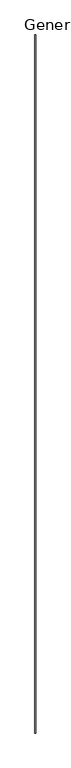
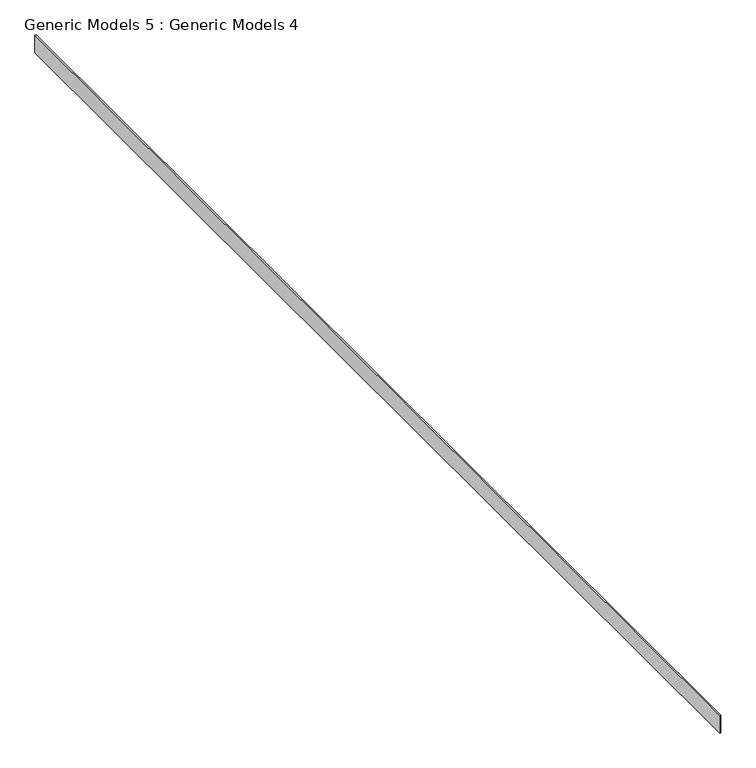
"""IFC4 building model written with IfcOpenShell, lengths in millimetres: proxy geometry, Generic Models 5 : Generic Models 4."""

import ifcopenshell
import ifcopenshell.guid

model = None  # the IFC model being written
_history = None  # IfcOwnerHistory: only IFC2X3 demands one
_inside = {}  # id of a spatial element -> (the spatial element, [elements in it])
_under = {}  # id of a project, library or spatial element -> (it, [spatial elements below it])
_declared = {}  # id of a project -> (the project, [libraries it declares])
_typed = {}  # id of a type object -> (the type object, [elements of that type])
_made_of = {}  # id of a material, layer set ... -> (it, [elements and type objects made of it])


def new_model(schema):
    """Start an empty IFC model of exactly this schema.

    Asked for "IFC4X3", IfcOpenShell would pick the latest addendum, in which some entities
    have other attributes; the version numbers below select the first issue.
    IFC2X3 requires an IfcOwnerHistory on every rooted entity: one is made here for all.
    """
    global model, _history
    if schema == "IFC4X3":
        model = ifcopenshell.file(schema_version=(4, 3, 0, 0))
    else:
        model = ifcopenshell.file(schema=schema)
    _inside.clear()
    _under.clear()
    _declared.clear()
    _typed.clear()
    _made_of.clear()
    _history = None
    if model.schema == "IFC2X3":
        org = make("IfcOrganization", Name="unknown")
        user = make(
            "IfcPersonAndOrganization",
            ThePerson=make("IfcPerson", FamilyName="unknown"),
            TheOrganization=org,
        )
        app = make(
            "IfcApplication",
            ApplicationDeveloper=org,
            Version="unknown",
            ApplicationFullName="unknown",
            ApplicationIdentifier="unknown",
        )
        _history = make(
            "IfcOwnerHistory",
            OwningUser=user,
            OwningApplication=app,
            ChangeAction="ADDED",
            CreationDate=0,
        )
    return model


def make(cls, **values):
    """One entity of the class cls with the attributes given. An attribute that is None is left unset."""
    return model.create_entity(
        cls, **{name: value for name, value in values.items() if value is not None}
    )


def rooted(cls, **values):
    """An entity with a GlobalId (a new one), such as an element, a storey or a relation."""
    return make(cls, GlobalId=ifcopenshell.guid.new(), OwnerHistory=_history, **values)


def si_unit(unit_type, name, prefix=None):
    """IfcSIUnit, for example si_unit("LENGTHUNIT", "METRE", prefix="MILLI")."""
    return make("IfcSIUnit", UnitType=unit_type, Prefix=prefix, Name=name)


def assignment(units):
    """IfcUnitAssignment: the units of a project."""
    return None if units is None else make("IfcUnitAssignment", Units=units)


def point(xyz):
    """IfcCartesianPoint."""
    return None if xyz is None else make("IfcCartesianPoint", Coordinates=xyz)


def direction(xyz):
    """IfcDirection."""
    return None if xyz is None else make("IfcDirection", DirectionRatios=xyz)


def frame(location, z_axis=None, x_axis=None):
    """IfcAxis2Placement3D, a coordinate frame: its origin and axes. An axis left out is left unset."""
    return make(
        "IfcAxis2Placement3D",
        Location=point(location),
        Axis=direction(z_axis),
        RefDirection=direction(x_axis),
    )


def origin():
    """The frame at (0, 0, 0) with its axes left unset."""
    return frame((0.0, 0.0, 0.0))


def place(relative_to, where):
    """IfcLocalPlacement: puts the frame where relative to a parent placement (None: the world)."""
    return make(
        "IfcLocalPlacement", PlacementRelTo=relative_to, RelativePlacement=where
    )


def context(
    kind, dimensions, precision=None, world=None, true_north=None, identifier=None
):
    """IfcGeometricRepresentationContext, for example the 3D "Model" context."""
    return make(
        "IfcGeometricRepresentationContext",
        ContextIdentifier=identifier,
        ContextType=kind,
        CoordinateSpaceDimension=dimensions,
        Precision=precision,
        WorldCoordinateSystem=world,
        TrueNorth=true_north,
    )


def project(units=None, contexts=None):
    """IfcProject with its units and contexts."""
    return rooted(
        "IfcProject",
        Name="project",
        RepresentationContexts=contexts,
        UnitsInContext=assignment(units),
    )


def spatial(cls, under=None, at=None, **own):
    """A site, building, storey or space (cls), placed at a placement, below another one or the project."""
    s = rooted(cls, ObjectPlacement=at, **own)
    if under is not None:
        _under.setdefault(under.id(), (under, []))[1].append(s)
    return s


def polyline(points):
    """IfcPolyline through the points."""
    return make("IfcPolyline", Points=[point(p) for p in points])


def outline(outer, holes=None, kind="AREA"):
    """IfcArbitraryClosedProfileDef: a profile drawn as a closed curve; with holes, ...WithVoids."""
    if holes is None:
        return make("IfcArbitraryClosedProfileDef", ProfileType=kind, OuterCurve=outer)
    return make(
        "IfcArbitraryProfileDefWithVoids",
        ProfileType=kind,
        OuterCurve=outer,
        InnerCurves=holes,
    )


def extrude(swept, where, along, depth):
    """IfcExtrudedAreaSolid: the profile swept, set in the frame where, extruded along a direction by depth."""
    return make(
        "IfcExtrudedAreaSolid",
        SweptArea=swept,
        Position=where,
        ExtrudedDirection=direction(along),
        Depth=depth,
    )


def shape(context_of_items, identifier, shape_type, items):
    """IfcShapeRepresentation: the items that make up one representation, for example the "Body"."""
    return make(
        "IfcShapeRepresentation",
        ContextOfItems=context_of_items,
        RepresentationIdentifier=identifier,
        RepresentationType=shape_type,
        Items=items,
    )


def source(mapping_origin, context_of_items, identifier, shape_type, items):
    """IfcRepresentationMap: a shape defined once, which mapped items show again and again."""
    return make(
        "IfcRepresentationMap",
        MappingOrigin=mapping_origin,
        MappedRepresentation=shape(context_of_items, identifier, shape_type, items),
    )


def transform(
    local_origin,
    x_axis=None,
    y_axis=None,
    z_axis=None,
    scale=None,
    scale2=None,
    scale3=None,
    uniform=True,
):
    """IfcCartesianTransformationOperator3D, or its non-uniform kind. x_axis, y_axis, z_axis: its Axis1, 2, 3."""
    if uniform:
        return make(
            "IfcCartesianTransformationOperator3D",
            Axis1=direction(x_axis),
            Axis2=direction(y_axis),
            LocalOrigin=point(local_origin),
            Scale=scale,
            Axis3=direction(z_axis),
        )
    return make(
        "IfcCartesianTransformationOperator3DnonUniform",
        Axis1=direction(x_axis),
        Axis2=direction(y_axis),
        LocalOrigin=point(local_origin),
        Scale=scale,
        Axis3=direction(z_axis),
        Scale2=scale2,
        Scale3=scale3,
    )


def mapped(mapping_source, mapping_target):
    """IfcMappedItem: shows the shape of a source again, moved by a transform."""
    return make(
        "IfcMappedItem", MappingSource=mapping_source, MappingTarget=mapping_target
    )


def made_of(thing, what):
    """Note that an element or type object is made of a material, layer set ...; save() writes the relation."""
    if what is not None:
        _made_of.setdefault(what.id(), (what, []))[1].append(thing)
    return thing


def element(
    cls,
    number,
    at=None,
    inside=None,
    cuts=None,
    type_object=None,
    material=None,
    context=None,
    identifier="Body",
    shape_type=None,
    held_by="IfcProductDefinitionShape",
    body=None,
    shapes=None,
    **own,
):
    """One element of the class cls, such as IfcWall. Its Tag is "e" and its number.

    at: its placement. inside: the storey or other place that contains it. cuts: it is an
    opening in that element (IfcRelVoidsElement). A single representation is given by context,
    identifier, shape_type and body (its items); several are given by shapes. held_by: the class
    of the entity that holds the representations. save() writes the other relations.
    """
    e = rooted(cls, Tag="e%d" % number, ObjectPlacement=at, **own)
    if body is not None:
        shapes = [shape(context, identifier, shape_type, body)]
    if shapes is not None:
        e.Representation = make(held_by, Representations=shapes)
    if inside is not None:
        _inside.setdefault(inside.id(), (inside, []))[1].append(e)
    if cuts is not None:
        rooted(
            "IfcRelVoidsElement", RelatingBuildingElement=cuts, RelatedOpeningElement=e
        )
    if type_object is not None:
        _typed.setdefault(type_object.id(), (type_object, []))[1].append(e)
    return made_of(e, material)


def aggregate(whole, parts):
    """IfcRelAggregates: a whole, such as a stair, and the parts it consists of."""
    return rooted("IfcRelAggregates", RelatingObject=whole, RelatedObjects=parts)


def save(model, path):
    """Write the relations noted so far, then the file.

    IfcRelAggregates (storeys below a building ...), IfcRelContainedInSpatialStructure (elements
    in a storey), IfcRelDefinesByType, IfcRelAssociatesMaterial and IfcRelDeclares: one each for
    every whole, place, type object, material and project.
    """
    for whole, parts in _under.values():
        aggregate(whole, parts)
    for where, things in _inside.values():
        rooted(
            "IfcRelContainedInSpatialStructure",
            RelatedElements=things,
            RelatingStructure=where,
        )
    for kind, things in _typed.values():
        rooted("IfcRelDefinesByType", RelatedObjects=things, RelatingType=kind)
    for what, things in _made_of.values():
        rooted("IfcRelAssociatesMaterial", RelatedObjects=things, RelatingMaterial=what)
    for by, libraries in _declared.values():
        rooted("IfcRelDeclares", RelatingContext=by, RelatedDefinitions=libraries)
    model.write(path)


def generic_models_5_generic_models_4_59b52fcf(model_context):
    return source(origin(), model_context, "Body", "SweptSolid", [
        extrude(outline(polyline([(8436.6513263, -6864.9230338), (8417.6013263, -6864.9230338), (8417.6013263, 11778.6769662), (8436.6513263, 11778.6769662), (8436.6513263, -6864.9230338)])), frame((0.0, 0.0, 126802.991198), z_axis=(0.0, 0.0, 1.0), x_axis=(1.0, 0.0, 0.0)), (0.0, 0.0, 1.0), 290.0279303),
    ])


if __name__ == "__main__":
    model = new_model("IFC4")
    model_context = context("Model", 3, world=origin())
    ifc_project = project(units=[si_unit("LENGTHUNIT", "METRE", prefix="MILLI")], contexts=[model_context])
    site = spatial("IfcSite", under=ifc_project)
    building = spatial("IfcBuilding", under=site)
    placement = place(None, origin())
    generic_models_5_generic_models_4_shape = generic_models_5_generic_models_4_59b52fcf(model_context)
    element("IfcBuildingElementProxy", 1, Name="Generic Models 5 : Generic Models 4", ObjectType="Generic Models 5 : Generic Models 4", at=placement, inside=building, context=model_context, shape_type="MappedRepresentation", body=[
        mapped(generic_models_5_generic_models_4_shape, transform((0.0, 0.0, 0.0), x_axis=(1.0, 0.0, 0.0), y_axis=(0.0, 1.0, 0.0), z_axis=(0.0, 0.0, 1.0))),
    ])
    save(model, "model.ifc")

# Revit data of these elements
# Element 1 (IfcBuildingElementProxy, "Generic Models 5 : Generic Models 4")
#   Materials on its faces: "_CDX PLYWOOD - SEE STRUCT DWGs"
# Materials
#   "_CDX PLYWOOD - SEE STRUCT DWGs": class "Generic", colour RGB 98 75 74, transparency 0, Cost = 0
